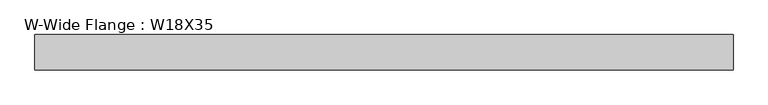
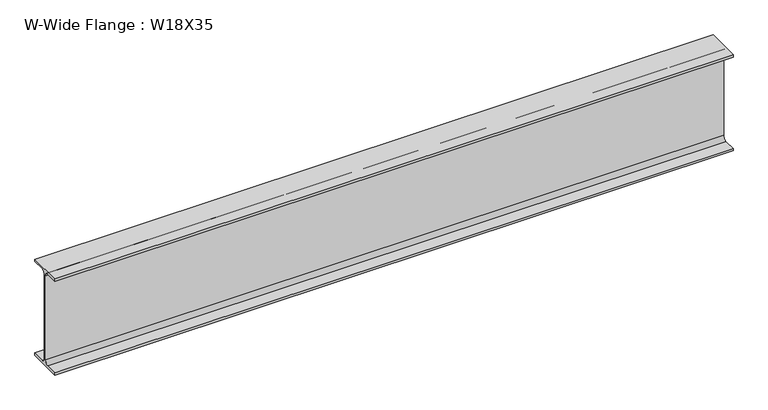
"""IFC4 building model written with IfcOpenShell, lengths in millimetres: beam geometry, W-Wide Flange : W18X35."""

import ifcopenshell
import ifcopenshell.guid

model = None  # the IFC model being written
_history = None  # IfcOwnerHistory: only IFC2X3 demands one
_inside = {}  # id of a spatial element -> (the spatial element, [elements in it])
_under = {}  # id of a project, library or spatial element -> (it, [spatial elements below it])
_declared = {}  # id of a project -> (the project, [libraries it declares])
_typed = {}  # id of a type object -> (the type object, [elements of that type])
_made_of = {}  # id of a material, layer set ... -> (it, [elements and type objects made of it])


def new_model(schema):
    """Start an empty IFC model of exactly this schema.

    Asked for "IFC4X3", IfcOpenShell would pick the latest addendum, in which some entities
    have other attributes; the version numbers below select the first issue.
    IFC2X3 requires an IfcOwnerHistory on every rooted entity: one is made here for all.
    """
    global model, _history
    if schema == "IFC4X3":
        model = ifcopenshell.file(schema_version=(4, 3, 0, 0))
    else:
        model = ifcopenshell.file(schema=schema)
    _inside.clear()
    _under.clear()
    _declared.clear()
    _typed.clear()
    _made_of.clear()
    _history = None
    if model.schema == "IFC2X3":
        org = make("IfcOrganization", Name="unknown")
        user = make(
            "IfcPersonAndOrganization",
            ThePerson=make("IfcPerson", FamilyName="unknown"),
            TheOrganization=org,
        )
        app = make(
            "IfcApplication",
            ApplicationDeveloper=org,
            Version="unknown",
            ApplicationFullName="unknown",
            ApplicationIdentifier="unknown",
        )
        _history = make(
            "IfcOwnerHistory",
            OwningUser=user,
            OwningApplication=app,
            ChangeAction="ADDED",
            CreationDate=0,
        )
    return model


def make(cls, **values):
    """One entity of the class cls with the attributes given. An attribute that is None is left unset."""
    return model.create_entity(
        cls, **{name: value for name, value in values.items() if value is not None}
    )


def rooted(cls, **values):
    """An entity with a GlobalId (a new one), such as an element, a storey or a relation."""
    return make(cls, GlobalId=ifcopenshell.guid.new(), OwnerHistory=_history, **values)


def si_unit(unit_type, name, prefix=None):
    """IfcSIUnit, for example si_unit("LENGTHUNIT", "METRE", prefix="MILLI")."""
    return make("IfcSIUnit", UnitType=unit_type, Prefix=prefix, Name=name)


def assignment(units):
    """IfcUnitAssignment: the units of a project."""
    return None if units is None else make("IfcUnitAssignment", Units=units)


def point(xyz):
    """IfcCartesianPoint."""
    return None if xyz is None else make("IfcCartesianPoint", Coordinates=xyz)


def direction(xyz):
    """IfcDirection."""
    return None if xyz is None else make("IfcDirection", DirectionRatios=xyz)


def frame(location, z_axis=None, x_axis=None):
    """IfcAxis2Placement3D, a coordinate frame: its origin and axes. An axis left out is left unset."""
    return make(
        "IfcAxis2Placement3D",
        Location=point(location),
        Axis=direction(z_axis),
        RefDirection=direction(x_axis),
    )


def frame_2d(location, x_axis=None):
    """IfcAxis2Placement2D, a coordinate frame in the plane: its origin and x axis."""
    return make(
        "IfcAxis2Placement2D", Location=point(location), RefDirection=direction(x_axis)
    )


def origin():
    """The frame at (0, 0, 0) with its axes left unset."""
    return frame((0.0, 0.0, 0.0))


def place(relative_to, where):
    """IfcLocalPlacement: puts the frame where relative to a parent placement (None: the world)."""
    return make(
        "IfcLocalPlacement", PlacementRelTo=relative_to, RelativePlacement=where
    )


def context(
    kind, dimensions, precision=None, world=None, true_north=None, identifier=None
):
    """IfcGeometricRepresentationContext, for example the 3D "Model" context."""
    return make(
        "IfcGeometricRepresentationContext",
        ContextIdentifier=identifier,
        ContextType=kind,
        CoordinateSpaceDimension=dimensions,
        Precision=precision,
        WorldCoordinateSystem=world,
        TrueNorth=true_north,
    )


def project(units=None, contexts=None):
    """IfcProject with its units and contexts."""
    return rooted(
        "IfcProject",
        Name="project",
        RepresentationContexts=contexts,
        UnitsInContext=assignment(units),
    )


def spatial(cls, under=None, at=None, **own):
    """A site, building, storey or space (cls), placed at a placement, below another one or the project."""
    s = rooted(cls, ObjectPlacement=at, **own)
    if under is not None:
        _under.setdefault(under.id(), (under, []))[1].append(s)
    return s


def polyline(points):
    """IfcPolyline through the points."""
    return make("IfcPolyline", Points=[point(p) for p in points])


def circle_curve(where, radius):
    """IfcCircle in the frame where."""
    return make("IfcCircle", Position=where, Radius=radius)


def trimmed(basis, trim1, trim2, sense, master):
    """IfcTrimmedCurve: the piece of a basis curve between two trims."""
    return make(
        "IfcTrimmedCurve",
        BasisCurve=basis,
        Trim1=trim1,
        Trim2=trim2,
        SenseAgreement=sense,
        MasterRepresentation=master,
    )


def segment(curve, same_sense, transition):
    """IfcCompositeCurveSegment."""
    return make(
        "IfcCompositeCurveSegment",
        Transition=transition,
        SameSense=same_sense,
        ParentCurve=curve,
    )


def composite_curve(segments, self_intersect=None):
    """IfcCompositeCurve: segments joined end to end."""
    return make("IfcCompositeCurve", Segments=segments, SelfIntersect=self_intersect)


def outline(outer, holes=None, kind="AREA"):
    """IfcArbitraryClosedProfileDef: a profile drawn as a closed curve; with holes, ...WithVoids."""
    if holes is None:
        return make("IfcArbitraryClosedProfileDef", ProfileType=kind, OuterCurve=outer)
    return make(
        "IfcArbitraryProfileDefWithVoids",
        ProfileType=kind,
        OuterCurve=outer,
        InnerCurves=holes,
    )


def extrude(swept, where, along, depth):
    """IfcExtrudedAreaSolid: the profile swept, set in the frame where, extruded along a direction by depth."""
    return make(
        "IfcExtrudedAreaSolid",
        SweptArea=swept,
        Position=where,
        ExtrudedDirection=direction(along),
        Depth=depth,
    )


def shape(context_of_items, identifier, shape_type, items):
    """IfcShapeRepresentation: the items that make up one representation, for example the "Body"."""
    return make(
        "IfcShapeRepresentation",
        ContextOfItems=context_of_items,
        RepresentationIdentifier=identifier,
        RepresentationType=shape_type,
        Items=items,
    )


def source(mapping_origin, context_of_items, identifier, shape_type, items):
    """IfcRepresentationMap: a shape defined once, which mapped items show again and again."""
    return make(
        "IfcRepresentationMap",
        MappingOrigin=mapping_origin,
        MappedRepresentation=shape(context_of_items, identifier, shape_type, items),
    )


def transform(
    local_origin,
    x_axis=None,
    y_axis=None,
    z_axis=None,
    scale=None,
    scale2=None,
    scale3=None,
    uniform=True,
):
    """IfcCartesianTransformationOperator3D, or its non-uniform kind. x_axis, y_axis, z_axis: its Axis1, 2, 3."""
    if uniform:
        return make(
            "IfcCartesianTransformationOperator3D",
            Axis1=direction(x_axis),
            Axis2=direction(y_axis),
            LocalOrigin=point(local_origin),
            Scale=scale,
            Axis3=direction(z_axis),
        )
    return make(
        "IfcCartesianTransformationOperator3DnonUniform",
        Axis1=direction(x_axis),
        Axis2=direction(y_axis),
        LocalOrigin=point(local_origin),
        Scale=scale,
        Axis3=direction(z_axis),
        Scale2=scale2,
        Scale3=scale3,
    )


def mapped(mapping_source, mapping_target):
    """IfcMappedItem: shows the shape of a source again, moved by a transform."""
    return make(
        "IfcMappedItem", MappingSource=mapping_source, MappingTarget=mapping_target
    )


def made_of(thing, what):
    """Note that an element or type object is made of a material, layer set ...; save() writes the relation."""
    if what is not None:
        _made_of.setdefault(what.id(), (what, []))[1].append(thing)
    return thing


def element(
    cls,
    number,
    at=None,
    inside=None,
    cuts=None,
    type_object=None,
    material=None,
    context=None,
    identifier="Body",
    shape_type=None,
    held_by="IfcProductDefinitionShape",
    body=None,
    shapes=None,
    **own,
):
    """One element of the class cls, such as IfcWall. Its Tag is "e" and its number.

    at: its placement. inside: the storey or other place that contains it. cuts: it is an
    opening in that element (IfcRelVoidsElement). A single representation is given by context,
    identifier, shape_type and body (its items); several are given by shapes. held_by: the class
    of the entity that holds the representations. save() writes the other relations.
    """
    e = rooted(cls, Tag="e%d" % number, ObjectPlacement=at, **own)
    if body is not None:
        shapes = [shape(context, identifier, shape_type, body)]
    if shapes is not None:
        e.Representation = make(held_by, Representations=shapes)
    if inside is not None:
        _inside.setdefault(inside.id(), (inside, []))[1].append(e)
    if cuts is not None:
        rooted(
            "IfcRelVoidsElement", RelatingBuildingElement=cuts, RelatedOpeningElement=e
        )
    if type_object is not None:
        _typed.setdefault(type_object.id(), (type_object, []))[1].append(e)
    return made_of(e, material)


def aggregate(whole, parts):
    """IfcRelAggregates: a whole, such as a stair, and the parts it consists of."""
    return rooted("IfcRelAggregates", RelatingObject=whole, RelatedObjects=parts)


def save(model, path):
    """Write the relations noted so far, then the file.

    IfcRelAggregates (storeys below a building ...), IfcRelContainedInSpatialStructure (elements
    in a storey), IfcRelDefinesByType, IfcRelAssociatesMaterial and IfcRelDeclares: one each for
    every whole, place, type object, material and project.
    """
    for whole, parts in _under.values():
        aggregate(whole, parts)
    for where, things in _inside.values():
        rooted(
            "IfcRelContainedInSpatialStructure",
            RelatedElements=things,
            RelatingStructure=where,
        )
    for kind, things in _typed.values():
        rooted("IfcRelDefinesByType", RelatedObjects=things, RelatingType=kind)
    for what, things in _made_of.values():
        rooted("IfcRelAssociatesMaterial", RelatedObjects=things, RelatingMaterial=what)
    for by, libraries in _declared.values():
        rooted("IfcRelDeclares", RelatingContext=by, RelatedDefinitions=libraries)
    model.write(path)


def w_wide_flange_w18x35_0a789f63(model_context):
    return source(origin(), model_context, "Body", "SweptSolid", [
        extrude(outline(composite_curve([segment(polyline([(76.2, -213.995), (76.2, -224.79), (-76.2, -224.79), (-76.2, -213.995), (-21.59, -213.995)]), True, "CONTINUOUS"), segment(trimmed(circle_curve(frame_2d((-21.59, -196.215)), 17.78), [point((-21.59, -213.995))], [point((-3.81, -196.215))], True, "CARTESIAN"), True, "CONTINUOUS"), segment(polyline([(-3.81, -196.215), (-3.81, 196.215)]), True, "CONTINUOUS"), segment(trimmed(circle_curve(frame_2d((-21.59, 196.215)), 17.78), [point((-3.81, 196.215))], [point((-21.59, 213.995))], True, "CARTESIAN"), True, "CONTINUOUS"), segment(polyline([(-21.59, 213.995), (-76.2, 213.995), (-76.2, 224.79), (76.2, 224.79), (76.2, 213.995), (21.59, 213.995)]), True, "CONTINUOUS"), segment(trimmed(circle_curve(frame_2d((21.59, 196.215)), 17.78), [point((21.59, 213.995))], [point((3.81, 196.215))], True, "CARTESIAN"), True, "CONTINUOUS"), segment(polyline([(3.81, 196.215), (3.81, -196.215)]), True, "CONTINUOUS"), segment(trimmed(circle_curve(frame_2d((21.59, -196.215)), 17.78), [point((3.81, -196.215))], [point((21.59, -213.995))], True, "CARTESIAN"), True, "CONTINUOUS"), segment(polyline([(21.59, -213.995), (76.2, -213.995)]), True, "CONTINUOUS")], self_intersect=False)), frame((-1474.0428396, 0.0, 0.0), z_axis=(1.0, 0.0, 0.0), x_axis=(0.0, 1.0, 0.0)), (0.0, 0.0, 1.0), 2995.8024999),
    ])


if __name__ == "__main__":
    model = new_model("IFC4")
    model_context = context("Model", 3, world=origin())
    ifc_project = project(units=[si_unit("LENGTHUNIT", "METRE", prefix="MILLI")], contexts=[model_context])
    site = spatial("IfcSite", under=ifc_project)
    building = spatial("IfcBuilding", under=site)
    placement = place(None, origin())
    w_wide_flange_w18x35_shape = w_wide_flange_w18x35_0a789f63(model_context)
    element("IfcBeam", 1, ObjectType="W-Wide Flange : W18X35", at=placement, inside=building, context=model_context, shape_type="MappedRepresentation", body=[
        mapped(w_wide_flange_w18x35_shape, transform((0.0, 0.0, 0.0), x_axis=(1.0, 0.0, 0.0), y_axis=(0.0, 1.0, 0.0), z_axis=(0.0, 0.0, 1.0))),
    ])
    save(model, "model.ifc")

# Revit data of these elements
# Type "W-Wide Flange : W18X35"
#   Assembly Code = "B10"
#   W = 35
#   Length [instance default] = 5' - 0"
#   bf = 0' - 6"
#   d = 1' - 5.7"
#   k = 0' - 1 1/8"
#   k2 = 0' - 0.7"
#   tf = 0' - 0.425"
#   tw = 0' - 0.3"
#   A = 0.0715278 SF
#   Structural Material [instance default] = Steel ASTM A992
# Element 1 (IfcBeam, "W-Wide Flange : W18X35")
#   Structural Material = Steel ASTM A36
#   Materials on its faces: "Steel ASTM A36"
# Materials
#   "Steel ASTM A992": class "Metal", colour RGB 199 199 199, transparency 0, Description = "Structural steel 50ksi", Cost = 0
#   "Steel ASTM A36": class "Metal", colour RGB 199 199 199, transparency 0, Description = "Structural steel, ASTM A36 Grade B, mill finish", Cost = 0
